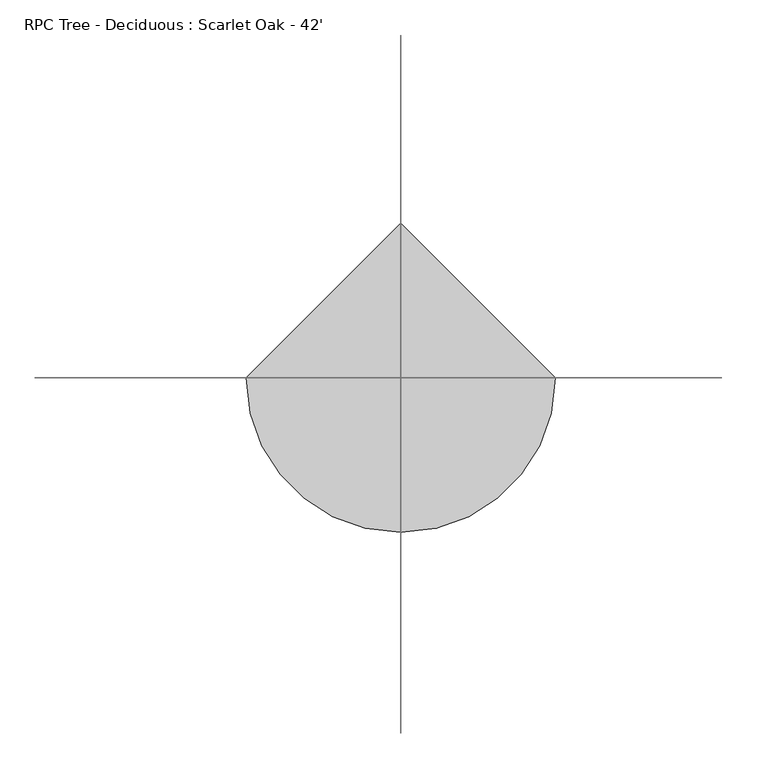
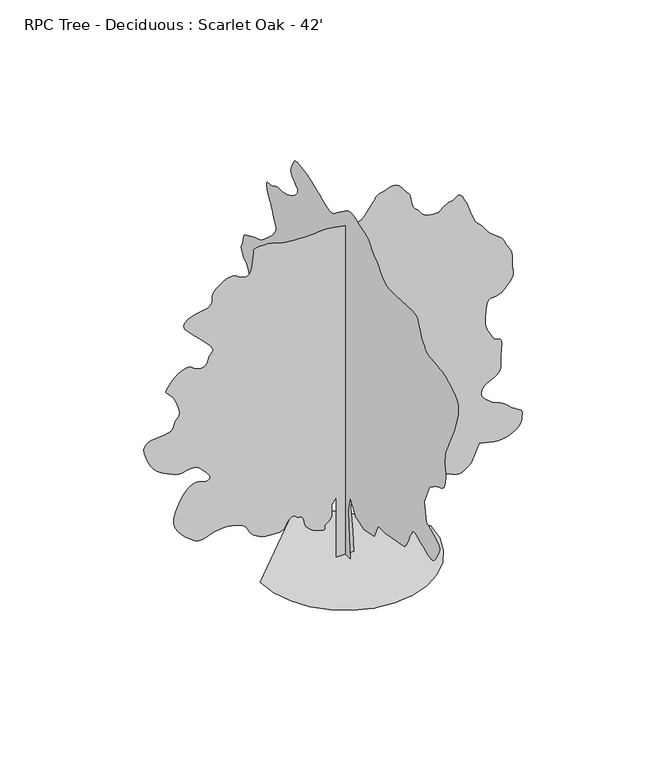
"""IFC4 building model written with IfcOpenShell, lengths in millimetres: geographic element geometry, RPC Tree - Deciduous : Scarlet Oak - 42'."""

import ifcopenshell
import ifcopenshell.guid

model = None  # the IFC model being written
_history = None  # IfcOwnerHistory: only IFC2X3 demands one
_inside = {}  # id of a spatial element -> (the spatial element, [elements in it])
_under = {}  # id of a project, library or spatial element -> (it, [spatial elements below it])
_declared = {}  # id of a project -> (the project, [libraries it declares])
_typed = {}  # id of a type object -> (the type object, [elements of that type])
_made_of = {}  # id of a material, layer set ... -> (it, [elements and type objects made of it])


def new_model(schema):
    """Start an empty IFC model of exactly this schema.

    Asked for "IFC4X3", IfcOpenShell would pick the latest addendum, in which some entities
    have other attributes; the version numbers below select the first issue.
    IFC2X3 requires an IfcOwnerHistory on every rooted entity: one is made here for all.
    """
    global model, _history
    if schema == "IFC4X3":
        model = ifcopenshell.file(schema_version=(4, 3, 0, 0))
    else:
        model = ifcopenshell.file(schema=schema)
    _inside.clear()
    _under.clear()
    _declared.clear()
    _typed.clear()
    _made_of.clear()
    _history = None
    if model.schema == "IFC2X3":
        org = make("IfcOrganization", Name="unknown")
        user = make(
            "IfcPersonAndOrganization",
            ThePerson=make("IfcPerson", FamilyName="unknown"),
            TheOrganization=org,
        )
        app = make(
            "IfcApplication",
            ApplicationDeveloper=org,
            Version="unknown",
            ApplicationFullName="unknown",
            ApplicationIdentifier="unknown",
        )
        _history = make(
            "IfcOwnerHistory",
            OwningUser=user,
            OwningApplication=app,
            ChangeAction="ADDED",
            CreationDate=0,
        )
    return model


def make(cls, **values):
    """One entity of the class cls with the attributes given. An attribute that is None is left unset."""
    return model.create_entity(
        cls, **{name: value for name, value in values.items() if value is not None}
    )


def rooted(cls, **values):
    """An entity with a GlobalId (a new one), such as an element, a storey or a relation."""
    return make(cls, GlobalId=ifcopenshell.guid.new(), OwnerHistory=_history, **values)


def si_unit(unit_type, name, prefix=None):
    """IfcSIUnit, for example si_unit("LENGTHUNIT", "METRE", prefix="MILLI")."""
    return make("IfcSIUnit", UnitType=unit_type, Prefix=prefix, Name=name)


def assignment(units):
    """IfcUnitAssignment: the units of a project."""
    return None if units is None else make("IfcUnitAssignment", Units=units)


def point(xyz):
    """IfcCartesianPoint."""
    return None if xyz is None else make("IfcCartesianPoint", Coordinates=xyz)


def direction(xyz):
    """IfcDirection."""
    return None if xyz is None else make("IfcDirection", DirectionRatios=xyz)


def frame(location, z_axis=None, x_axis=None):
    """IfcAxis2Placement3D, a coordinate frame: its origin and axes. An axis left out is left unset."""
    return make(
        "IfcAxis2Placement3D",
        Location=point(location),
        Axis=direction(z_axis),
        RefDirection=direction(x_axis),
    )


def origin():
    """The frame at (0, 0, 0) with its axes left unset."""
    return frame((0.0, 0.0, 0.0))


def place(relative_to, where):
    """IfcLocalPlacement: puts the frame where relative to a parent placement (None: the world)."""
    return make(
        "IfcLocalPlacement", PlacementRelTo=relative_to, RelativePlacement=where
    )


def context(
    kind, dimensions, precision=None, world=None, true_north=None, identifier=None
):
    """IfcGeometricRepresentationContext, for example the 3D "Model" context."""
    return make(
        "IfcGeometricRepresentationContext",
        ContextIdentifier=identifier,
        ContextType=kind,
        CoordinateSpaceDimension=dimensions,
        Precision=precision,
        WorldCoordinateSystem=world,
        TrueNorth=true_north,
    )


def project(units=None, contexts=None):
    """IfcProject with its units and contexts."""
    return rooted(
        "IfcProject",
        Name="project",
        RepresentationContexts=contexts,
        UnitsInContext=assignment(units),
    )


def spatial(cls, under=None, at=None, **own):
    """A site, building, storey or space (cls), placed at a placement, below another one or the project."""
    s = rooted(cls, ObjectPlacement=at, **own)
    if under is not None:
        _under.setdefault(under.id(), (under, []))[1].append(s)
    return s


def point_list(points):
    """IfcCartesianPointList2D or 3D."""
    cls = (
        "IfcCartesianPointList2D" if len(points[0]) == 2 else "IfcCartesianPointList3D"
    )
    return make(cls, CoordList=points)


def triangles(points, corners, closed=None, point_numbers=None):
    """IfcTriangulatedFaceSet: each triangle names its three corners, points numbered from 1."""
    return make(
        "IfcTriangulatedFaceSet",
        Coordinates=point_list(points),
        Closed=closed,
        CoordIndex=corners,
        PnIndex=point_numbers,
    )


def shape(context_of_items, identifier, shape_type, items):
    """IfcShapeRepresentation: the items that make up one representation, for example the "Body"."""
    return make(
        "IfcShapeRepresentation",
        ContextOfItems=context_of_items,
        RepresentationIdentifier=identifier,
        RepresentationType=shape_type,
        Items=items,
    )


def source(mapping_origin, context_of_items, identifier, shape_type, items):
    """IfcRepresentationMap: a shape defined once, which mapped items show again and again."""
    return make(
        "IfcRepresentationMap",
        MappingOrigin=mapping_origin,
        MappedRepresentation=shape(context_of_items, identifier, shape_type, items),
    )


def transform(
    local_origin,
    x_axis=None,
    y_axis=None,
    z_axis=None,
    scale=None,
    scale2=None,
    scale3=None,
    uniform=True,
):
    """IfcCartesianTransformationOperator3D, or its non-uniform kind. x_axis, y_axis, z_axis: its Axis1, 2, 3."""
    if uniform:
        return make(
            "IfcCartesianTransformationOperator3D",
            Axis1=direction(x_axis),
            Axis2=direction(y_axis),
            LocalOrigin=point(local_origin),
            Scale=scale,
            Axis3=direction(z_axis),
        )
    return make(
        "IfcCartesianTransformationOperator3DnonUniform",
        Axis1=direction(x_axis),
        Axis2=direction(y_axis),
        LocalOrigin=point(local_origin),
        Scale=scale,
        Axis3=direction(z_axis),
        Scale2=scale2,
        Scale3=scale3,
    )


def mapped(mapping_source, mapping_target):
    """IfcMappedItem: shows the shape of a source again, moved by a transform."""
    return make(
        "IfcMappedItem", MappingSource=mapping_source, MappingTarget=mapping_target
    )


def made_of(thing, what):
    """Note that an element or type object is made of a material, layer set ...; save() writes the relation."""
    if what is not None:
        _made_of.setdefault(what.id(), (what, []))[1].append(thing)
    return thing


def element(
    cls,
    number,
    at=None,
    inside=None,
    cuts=None,
    type_object=None,
    material=None,
    context=None,
    identifier="Body",
    shape_type=None,
    held_by="IfcProductDefinitionShape",
    body=None,
    shapes=None,
    **own,
):
    """One element of the class cls, such as IfcWall. Its Tag is "e" and its number.

    at: its placement. inside: the storey or other place that contains it. cuts: it is an
    opening in that element (IfcRelVoidsElement). A single representation is given by context,
    identifier, shape_type and body (its items); several are given by shapes. held_by: the class
    of the entity that holds the representations. save() writes the other relations.
    """
    e = rooted(cls, Tag="e%d" % number, ObjectPlacement=at, **own)
    if body is not None:
        shapes = [shape(context, identifier, shape_type, body)]
    if shapes is not None:
        e.Representation = make(held_by, Representations=shapes)
    if inside is not None:
        _inside.setdefault(inside.id(), (inside, []))[1].append(e)
    if cuts is not None:
        rooted(
            "IfcRelVoidsElement", RelatingBuildingElement=cuts, RelatedOpeningElement=e
        )
    if type_object is not None:
        _typed.setdefault(type_object.id(), (type_object, []))[1].append(e)
    return made_of(e, material)


def aggregate(whole, parts):
    """IfcRelAggregates: a whole, such as a stair, and the parts it consists of."""
    return rooted("IfcRelAggregates", RelatingObject=whole, RelatedObjects=parts)


def save(model, path):
    """Write the relations noted so far, then the file.

    IfcRelAggregates (storeys below a building ...), IfcRelContainedInSpatialStructure (elements
    in a storey), IfcRelDefinesByType, IfcRelAssociatesMaterial and IfcRelDeclares: one each for
    every whole, place, type object, material and project.
    """
    for whole, parts in _under.values():
        aggregate(whole, parts)
    for where, things in _inside.values():
        rooted(
            "IfcRelContainedInSpatialStructure",
            RelatedElements=things,
            RelatingStructure=where,
        )
    for kind, things in _typed.values():
        rooted("IfcRelDefinesByType", RelatedObjects=things, RelatingType=kind)
    for what, things in _made_of.values():
        rooted("IfcRelAssociatesMaterial", RelatedObjects=things, RelatingMaterial=what)
    for by, libraries in _declared.values():
        rooted("IfcRelDeclares", RelatingContext=by, RelatedDefinitions=libraries)
    model.write(path)


def rpc_tree_deciduous_scarlet_oak_42_9b182cbb(model_context):
    return source(origin(), model_context, "Body", "Tessellation", [
        triangles([(0.0176667, 313.3908637, 0.0), (0.0176667, -300.6481277, 0.0), (0.0176667, -201.6098415, 1168.65294), (0.0176667, -181.8016574, 1723.2669067), (0.0176667, -300.6481277, 2238.2675938), (0.0176667, -617.5722605, 1723.2669067), (0.0176667, -1132.5703314, 1564.8060848), (0.0176667, -1726.8001213, 1703.4602669), (0.0176667, -1964.4925896, 2198.6516979), (0.0176667, -2380.4549904, 2198.6516979), (0.0176667, -3529.2988197, 2416.5375263), (0.0176667, -3571.5694954, 2467.5287453), (0.0176667, -3612.8163963, 2518.865728), (0.0176667, -3651.9637161, 2570.8942383), (0.0176667, -3687.9873894, 2623.969487), (0.0176667, -3719.8633507, 2678.4275002), (0.0176667, -3746.5419548, 2734.6266861), (0.0176667, -3766.9988457, 2792.8740028), (0.0176667, -3786.866819, 2852.8877815), (0.0176667, -3811.9324402, 2913.9259163), (0.0176667, -3841.3248322, 2975.8343468), (0.0176667, -3874.1736992, 3038.4340141), (0.0176667, -3909.6343254, 3101.5461502), (0.0176667, -3946.8099632, 3165.016404), (0.0176667, -3984.882058, 3228.6404274), (0.0176667, -4003.0091492, 3249.1996376), (0.0176667, -4028.0747704, 3265.7904854), (0.0176667, -4066.991581, 3274.393158), (0.0176667, -4126.698111, 3271.0392929), (0.0176667, -4214.133181, 3251.7599464), (0.0176667, -4336.2091599, 3212.5358871), (0.0176667, -4499.8648682, 3149.4240417), (0.0176667, -4672.6607162, 3075.1492149), (0.0176667, -4819.8023163, 3008.8625633), (0.0176667, -4944.7714325, 2956.0686928), (0.0176667, -5051.0248306, 2922.3492393), (0.0176667, -5142.0442749, 2913.2343887), (0.0176667, -5221.2603699, 2934.2546173), (0.0176667, -5292.1816223, 2990.9656906), (0.0176667, -5363.7423706, 3080.2954124), (0.0176667, -5437.7099487, 3189.0320892), (0.0176667, -5506.8388687, 3307.4725342), (0.0176667, -5563.8313202, 3425.9129791), (0.0176667, -5601.4168167, 3534.6496559), (0.0176667, -5612.3492889, 3624.0049576), (0.0176667, -5589.3065094, 3684.2236656), (0.0176667, -5533.0052948, 3729.5668282), (0.0176667, -5451.7404877, 3780.0820587), (0.0176667, -5349.7118317, 3834.9496399), (0.0176667, -5231.0155884, 3893.2736961), (0.0176667, -5099.8759186, 3954.2095116), (0.0176667, -4960.4152451, 4016.8603386), (0.0176667, -4816.8068596, 4080.3820427), (0.0176667, -4697.9568466, 4753.8484932), (0.0176667, -4995.0561539, 5447.1064682), (0.0176667, -5004.4270935, 5460.3434509), (0.0176667, -5018.9698105, 5476.4988602), (0.0176667, -5043.9328217, 5498.5690247), (0.0176667, -5084.4629059, 5529.4717896), (0.0176667, -5145.7824188, 5572.1267441), (0.0176667, -5233.1148788, 5629.5290543), (0.0176667, -5351.6064835, 5704.6233078), (0.0176667, -5480.1602646, 5772.6511322), (0.0176667, -5594.1457489, 5817.0984192), (0.0176667, -5693.5885162, 5853.2497009), (0.0176667, -5778.4885666, 5896.340094), (0.0176667, -5848.8209015, 5961.6029709), (0.0176667, -5904.609938, 6064.2717041), (0.0176667, -5945.8312592, 6219.6064087), (0.0176667, -5969.6931747, 6372.1755844), (0.0176667, -5976.5549652, 6470.0056595), (0.0176667, -5971.3064484, 6533.5267822), (0.0176667, -5958.7607025, 6583.1970062), (0.0176667, -5943.8087082, 6639.4476425), (0.0176667, -5931.2885422, 6722.7088394), (0.0176667, -5926.0400253, 6853.4648117), (0.0176667, -5927.8835175, 6997.7129837), (0.0176667, -5935.9737213, 7117.3568436), (0.0176667, -5954.1011032, 7226.6309875), (0.0176667, -5986.0793839, 7339.6950165), (0.0176667, -6035.7496078, 7470.7835266), (0.0176667, -6106.9010788, 7634.1061157), (0.0176667, -6203.3225189, 7843.8473831), (0.0176667, -6294.8797211, 8033.439299), (0.0176667, -6355.9178558, 8147.834642), (0.0176667, -6397.1897552, 8218.5762543), (0.0176667, -6429.4755753, 8277.1819794), (0.0176667, -6463.5019867, 8355.1946594), (0.0176667, -6509.9718246, 8484.1577179), (0.0176667, -6579.6896622, 8695.5634186), (0.0176667, -6654.8094955, 8940.125235), (0.0176667, -6705.3500153, 9150.7373795), (0.0176667, -6723.656456, 9332.2385101), (0.0176667, -6702.0984695, 9489.4934464), (0.0176667, -6633.0980301, 9627.3408463), (0.0176667, -6508.9992096, 9750.6205307), (0.0176667, -6322.1728226, 9864.2211548), (0.0176667, -6140.9019104, 9957.5968506), (0.0176667, -6021.6679092, 10021.8859497), (0.0176667, -5939.1485275, 10064.3101044), (0.0176667, -5868.0487976, 10092.2177032), (0.0176667, -5783.0970062, 10112.8292358), (0.0176667, -5658.9987671, 10133.4396057), (0.0176667, -5470.4567871, 10161.3472046), (0.0176667, -5268.216806, 10183.3400482), (0.0176667, -5111.3717285, 10191.8406921), (0.0176667, -4987.0938492, 10202.3888855), (0.0176667, -4882.5816238, 10230.6290222), (0.0176667, -4784.982058, 10292.127594), (0.0176667, -4681.493898, 10402.5034149), (0.0176667, -4559.2897293, 10577.2962341), (0.0176667, -4452.5756035, 10769.4740387), (0.0176667, -4389.5149178, 10923.9122864), (0.0176667, -4348.2938873, 11044.0165833), (0.0176667, -4307.0469864, 11133.2960175), (0.0176667, -4243.9863007, 11195.2038666), (0.0176667, -4137.2721748, 11233.1992218), (0.0176667, -3965.0652443, 11250.763266), (0.0176667, -3014.2904297, 11191.3378235), (0.0176667, -2839.0363014, 11194.4108917), (0.0176667, -2696.349662, 11194.0004517), (0.0176667, -2575.1186897, 11201.2209412), (0.0176667, -2464.3027794, 11227.1309875), (0.0176667, -2352.7906906, 11282.8694458), (0.0176667, -2229.4985069, 11379.4705261), (0.0176667, -2083.3375156, 11528.0707581), (0.0176667, -1942.4917522, 11678.1569458), (0.0176667, -1836.9835121, 11780.4158203), (0.0176667, -1758.5045815, 11847.7012482), (0.0176667, -1698.7339565, 11892.8147736), (0.0176667, -1649.3606621, 11928.556778), (0.0176667, -1602.0639851, 11967.7555481), (0.0176667, -1548.5328049, 12023.2626251), (0.0176667, -1497.1368141, 12088.8074615), (0.0176667, -1455.0938862, 12149.8444336), (0.0176667, -1412.3621922, 12206.7351471), (0.0176667, -1358.8872585, 12259.7853973), (0.0176667, -1284.6226055, 12309.4044617), (0.0176667, -1179.5189192, 12355.8992981), (0.0176667, -1033.5320452, 12399.6036072), (0.0176667, -869.6434296, 12447.7634583), (0.0176667, -716.8409832, 12501.1206665), (0.0176667, -574.0851983, 12550.3304535), (0.0176667, -440.341763, 12586.0212982), (0.0176667, -314.5660463, 12598.8484222), (0.0176667, -195.7190492, 12579.4414673), (0.0176667, -82.7633712, 12518.4544922), (0.0176667, 511.4674361, 12082.6880676), (0.0176667, 575.7980298, 12024.1335022), (0.0176667, 638.0522604, 11970.7762939), (0.0176667, 705.8469595, 11927.7882202), (0.0176667, 786.8119303, 11900.4189606), (0.0176667, 888.5641497, 11893.8379669), (0.0176667, 1018.7282976, 11913.2460846), (0.0176667, 1184.9289087, 11963.8371826), (0.0176667, 1373.534911, 12038.957016), (0.0176667, 1563.5259304, 12123.4483704), (0.0176667, 1751.4381523, 12209.6791534), (0.0176667, 1933.8071079, 12289.996344), (0.0176667, 2107.1689098, 12356.8213348), (0.0176667, 2268.0542931, 12402.4976166), (0.0176667, 2413.0043118, 12419.4210022), (0.0176667, 2544.8429214, 12428.6634613), (0.0176667, 2667.3156784, 12449.6842712), (0.0176667, 2778.3824455, 12472.4200928), (0.0176667, 2875.9049812, 12486.8599091), (0.0176667, 2957.8610252, 12482.9427063), (0.0176667, 3022.1248352, 12450.606308), (0.0176667, 3066.6488617, 12379.7873749), (0.0176667, 3106.4362587, 12290.8160614), (0.0176667, 3152.1122498, 12208.7582794), (0.0176667, 3195.0232933, 12130.8479187), (0.0176667, 3226.5152664, 12054.318869), (0.0176667, 3237.8831772, 11976.4340881), (0.0176667, 3220.4984825, 11894.3763062), (0.0176667, 3165.7076408, 11805.3794128), (0.0176667, 3081.8572357, 11723.8332275), (0.0176667, 2992.092366, 11659.9534058), (0.0176667, 2909.982843, 11604.7532867), (0.0176667, 2848.9961586, 11549.1938873), (0.0176667, 2822.6759628, 11484.2897095), (0.0176667, 2844.4900383, 11401.0285126), (0.0176667, 2928.0076149, 11290.3713135), (0.0176667, 3043.3244133, 11180.1233917), (0.0176667, 3152.0610901, 11099.7038818), (0.0176667, 3254.9091728, 11042.4550507), (0.0176667, 3352.5598984, 11001.8738068), (0.0176667, 3445.704213, 10971.3035797), (0.0176667, 3535.0595146, 10944.2412781), (0.0176667, 3621.2652992, 10914.0291687), (0.0176667, 3707.3690552, 10890.7561707), (0.0176667, 3795.9049301, 10883.0752441), (0.0176667, 3886.8473442, 10882.333429), (0.0176667, 3980.222168, 10879.8498596), (0.0176667, 4076.0294014, 10866.9715759), (0.0176667, 4174.2690445, 10835.0177124), (0.0176667, 4274.9152267, 10775.3887939), (0.0176667, 4378.9408539, 10722.4152832), (0.0176667, 4481.2000191, 10703.4176056), (0.0176667, 4572.7316414, 10698.9632263), (0.0176667, 4644.5228989, 10689.6684448), (0.0176667, 4687.5362617, 10656.1286316), (0.0176667, 4692.7850693, 10578.9089264), (0.0176667, 4651.2820793, 10438.6546967), (0.0176667, 4589.9369865, 10291.0520782), (0.0176667, 4539.012188, 10191.6093109), (0.0176667, 4494.308812, 10120.561322), (0.0176667, 4451.7053078, 10058.1918732), (0.0176667, 4407.0019318, 9984.7358917), (0.0176667, 4356.0515533, 9880.4538849), (0.0176667, 4294.7320404, 9725.5801987), (0.0176667, 4229.9301819, 9573.2412415), (0.0176667, 4174.1664345, 9477.02444), (0.0176667, 4131.5370598, 9417.880957), (0.0176667, 4106.2412201, 9376.7625366), (0.0176667, 4102.4263367, 9334.6197601), (0.0176667, 4124.265992, 9272.3526306), (0.0176667, 4175.8820274, 9170.9640518), (0.0176667, 4267.7717674, 9036.5728363), (0.0176667, 4396.7095367, 8893.8861969), (0.0176667, 4546.4626053, 8751.5320953), (0.0176667, 4700.6962143, 8618.1908157), (0.0176667, 4843.178215, 8502.5153183), (0.0176667, 4957.5729767, 8413.1858871), (0.0176667, 5027.6233521, 8358.830484), (0.0176667, 5089.8137421, 8324.829071), (0.0176667, 5183.1888565, 8290.4695404), (0.0176667, 5295.279689, 8255.4187729), (0.0176667, 5413.6172333, 8219.3186508), (0.0176667, 5525.7080658, 8181.8354736), (0.0176667, 5619.0831802, 8142.6367035), (0.0176667, 5681.2729889, 8101.3392242), (0.0176667, 5733.3500427, 8067.0308533), (0.0176667, 5799.6622742, 8042.7846588), (0.0176667, 5872.5293381, 8019.2297012), (0.0176667, 5944.3714645, 7986.9950409), (0.0176667, 6007.5606308, 7936.7614792), (0.0176667, 6054.4397461, 7859.1324966), (0.0176667, 6077.431366, 7744.7888947), (0.0176667, 6096.2499847, 7629.9325333), (0.0176667, 6128.5869644, 7548.6938873), (0.0176667, 6163.6888916, 7488.5777893), (0.0176667, 6190.8535126, 7437.1152328), (0.0176667, 6199.277417, 7381.8633728), (0.0176667, 6178.2571884, 7310.3026245), (0.0176667, 6117.0399948, 7209.9889801), (0.0176667, 6041.0492844, 7116.0255295), (0.0176667, 5979.6018723, 7059.8522141), (0.0176667, 5927.8579376, 7023.4183914), (0.0176667, 5880.9526611, 6988.7007431), (0.0176667, 5834.0729645, 6937.699205), (0.0176667, 5782.3290298, 6852.4148758), (0.0176667, 5720.8816177, 6714.7976944), (0.0176667, 5653.9037292, 6576.9502945), (0.0176667, 5592.4557358, 6490.0526917), (0.0176667, 5542.0942749, 6434.6729324), (0.0176667, 5508.3748215, 6391.4034805), (0.0176667, 5496.8278519, 6340.8885406), (0.0176667, 5512.9832611, 6263.6694168), (0.0176667, 5562.4232666, 6140.3897324), (0.0176667, 5628.0954208, 6005.5380798), (0.0176667, 5689.9271118, 5900.8462143), (0.0176667, 5749.0194351, 5817.6361771), (0.0176667, 5806.3450058, 5747.2271027), (0.0176667, 5863.0049194, 5680.9916107), (0.0176667, 5919.9973709, 5610.2499985), (0.0176667, 5978.3728775, 5526.348143), (0.0176667, 6046.1187424, 5443.5985428), (0.0176667, 6124.9511398, 5376.0828964), (0.0176667, 6206.5484848, 5314.8145432), (0.0176667, 6282.6153534, 5250.7556625), (0.0176667, 6344.8057434, 5174.9445923), (0.0176667, 6384.8236496, 5078.3179321), (0.0176667, 6394.3480682, 4951.9151825), (0.0176667, 6402.3615326, 4852.6511833), (0.0176667, 6431.8824051, 4819.9049263), (0.0176667, 6465.5506989, 4818.343103), (0.0176667, 6486.0587494, 4812.6335678), (0.0176667, 6476.0477325, 4767.4183044), (0.0176667, 6418.2611435, 4647.3648766), (0.0176667, 6295.3145782, 4417.1152679), (0.0176667, 6166.7613785, 4158.8557411), (0.0176667, 6089.1579758, 3968.8801277), (0.0176667, 6040.640007, 3832.9270889), (0.0176667, 5999.4186859, 3736.8381866), (0.0176667, 5943.629068, 3666.3782433), (0.0176667, 5851.4579498, 3607.3629501), (0.0176667, 5701.0903839, 3545.5824188), (0.0176667, 5527.4748184, 3495.4511765), (0.0176667, 5374.6748428, 3474.4309479), (0.0176667, 5234.3438736, 3472.8179649), (0.0176667, 5098.1859055, 3480.9087502), (0.0176667, 4957.8549362, 3488.9736649), (0.0176667, 4805.0549606, 3487.3606819), (0.0176667, 4631.4652657, 3466.3404533), (0.0176667, 4458.3362984, 3447.5221252), (0.0176667, 4308.7625793, 3451.5675179), (0.0176667, 4177.2133415, 3467.3900986), (0.0176667, 4058.1328194, 3483.9042068), (0.0176667, 3945.9908272, 3490.0233101), (0.0176667, 3835.2313087, 3474.6614571), (0.0176667, 3720.2984985, 3426.7324059), (0.0176667, 3610.3072472, 3375.7820274), (0.0176667, 3519.3389626, 3349.1034233), (0.0176667, 3449.5190964, 3332.1285873), (0.0176667, 3402.9213593, 3310.3145119), (0.0176667, 3381.6194618, 3269.0679016), (0.0176667, 3387.6874054, 3193.8969086), (0.0176667, 3423.1991913, 3070.1820763), (0.0176667, 3480.4733116, 2938.7610283), (0.0176667, 3549.1923729, 2845.7701927), (0.0176667, 3627.4614326, 2784.8599571), (0.0176667, 3713.3343887, 2749.5789711), (0.0176667, 3804.9171707, 2733.5255905), (0.0176667, 3900.3145454, 2730.2740448), (0.0176667, 3997.6068626, 2733.448851), (0.0176667, 4373.9740059, 2317.4992401), (0.0176667, 4403.4687172, 2270.6632908), (0.0176667, 4431.7603043, 2222.9646034), (0.0176667, 4457.6450615, 2173.5324463), (0.0176667, 4479.868705, 2121.4991398), (0.0176667, 4497.2533997, 2066.004126), (0.0176667, 4508.5698601, 2006.1771091), (0.0176667, 4512.6152527, 1941.1527351), (0.0176667, 4511.9240158, 1873.3554199), (0.0176667, 4507.0847763, 1806.2519577), (0.0176667, 4493.8992439, 1740.5362015), (0.0176667, 4468.2705757, 1676.8969173), (0.0176667, 4425.9996094, 1616.0304291), (0.0176667, 4362.9389236, 1558.6281189), (0.0176667, 4274.9152267, 1505.3836945), (0.0176667, 4190.9622116, 1460.165815), (0.0176667, 4131.9469185, 1424.9973221), (0.0176667, 4081.5854576, 1397.7989822), (0.0176667, 4023.5942299, 1376.4895271), (0.0176667, 3941.7149254, 1358.992194), (0.0176667, 3819.6389465, 1343.2258598), (0.0176667, 3641.0824036, 1327.1137619), (0.0176667, 3437.9721268, 1329.4230686), (0.0176667, 3250.8126205, 1364.996188), (0.0176667, 3076.1221207, 1425.8652924), (0.0176667, 2910.4438614, 1504.0548512), (0.0176667, 2750.3213676, 1591.6024143), (0.0176667, 2592.2472954, 1680.5352127), (0.0176667, 2432.8109516, 1762.8828026), (0.0176667, 2290.6338741, 1837.7823006), (0.0176667, 2180.6808472, 1908.5239128), (0.0176667, 2093.9423916, 1973.376931), (0.0176667, 2021.411063, 2030.6051239), (0.0176667, 1954.0772369, 2078.4780739), (0.0176667, 1882.9309982, 2115.2646366), (0.0176667, 1798.9653385, 2139.2293076), (0.0176667, 1706.624754, 2159.4404285), (0.0176667, 1615.6720207, 2184.5034336), (0.0176667, 1525.0649059, 2211.9936161), (0.0176667, 1433.7664089, 2239.4811825), (0.0176667, 1340.7321167, 2264.5441875), (0.0176667, 1244.9274994, 2284.7553085), (0.0176667, 1145.3130856, 2297.6899841), (0.0176667, 1043.4456116, 2304.4466938), (0.0176667, 941.5755941, 2308.0849892), (0.0176667, 839.7081202, 2309.1244606), (0.0176667, 737.8407188, 2308.0849892), (0.0176667, 635.9732449, 2305.4861652), (0.0176667, 534.1032274, 2301.8480152), (0.0176667, 432.2357898, 2297.6899841), (0.0176667, 234.1596897, 2000.5751255), (0.0176667, 194.5438665, 1544.999445), (287.211575, 0.0006153, 0.0094345), (-307.0182149, 0.0006153, 0.0094345), (-307.0182149, 0.0004871, 2178.8527611), (-465.4815439, 0.0004871, 1960.9695488), (-465.4815439, 0.0005127, 1723.2770805), (-461.8433212, 0.0005127, 1668.1278305), (-461.8433212, 0.0005127, 1613.1500816), (-469.1197666, 0.0005127, 1558.5205673), (-487.308264, 0.0005384, 1504.4107887), (-520.0521955, 0.0005384, 1450.9948631), (-570.9872043, 0.0005384, 1398.4416756), (-643.748933, 0.0005384, 1346.9305756), (-700.7467621, 0.0005384, 1293.4557873), (-716.5132416, 0.0005384, 1239.2870007), (-712.8750189, 0.0005384, 1191.0121857), (-711.6614302, 0.0005384, 1155.206159), (-734.7042824, 0.0005384, 1138.4590708), (-803.8278248, 0.0005384, 1147.3536587), (-940.8638643, 0.0005384, 1188.4698263), (-1097.1892788, 0.0005384, 1252.5136642), (-1214.0141247, 0.0005384, 1324.8708755), (-1297.9209217, 0.0005384, 1404.1613846), (-1355.4973492, 0.0005384, 1488.9925438), (-1393.3235287, 0.0005127, 1577.9815887), (-1417.9820526, 0.0005127, 1669.7434296), (-1436.0578388, 0.0005127, 1762.8929764), (-1440.6767429, 0.0005127, 1788.2427372), (-1447.5485619, 0.0005127, 1812.9011158), (-1458.9240303, 0.0005127, 1836.1770206), (-1477.0588245, 0.0005127, 1857.3687504), (-1504.1983017, 0.0005127, 1875.7903004), (-1542.6030796, 0.0005127, 1890.7476723), (-1594.5186607, 0.0005127, 1901.5471584), (-1646.4342419, 0.0005127, 1919.331102), (-1687.2611103, 0.0005127, 1949.2458458), (-1722.8930923, 0.0004871, 1981.5852962), (-1759.2163113, 0.0004871, 2006.6483013), (-1802.1247387, 0.0004871, 2014.733709), (-1857.5044979, 0.0004871, 1996.138187), (-1931.2494152, 0.0005127, 1941.1604382), (-1996.0996719, 0.0005127, 1864.2407146), (-2032.88638, 0.0005127, 1789.0516994), (-2059.6238468, 0.0005127, 1719.7541851), (-2094.3289959, 0.0005127, 1660.5031506), (-2155.0238377, 0.0005127, 1615.4620045), (-2259.7204994, 0.0005127, 1588.7809296), (-2426.4408463, 0.0005127, 1584.6230438), (-2610.6557648, 0.0005127, 1596.8664825), (-2760.2297745, 0.0005127, 1617.0776035), (-2881.7168358, 0.0005127, 1645.9528759), (-2981.7488113, 0.0005127, 1684.1810658), (-3066.8793709, 0.0005127, 1732.4584969), (-3143.6633469, 0.0005127, 1791.4788769), (-3218.7576004, 0.0005127, 1861.9312626), (-3282.4327835, 0.0005127, 1939.1966045), (-3328.1343544, 0.0004871, 2016.8126518), (-3366.8721062, 0.0004871, 2092.6929039), (-3409.782859, 0.0004871, 2164.7633595), (-3467.9278564, 0.0004871, 2230.9424595), (-3552.4183388, 0.0004871, 2289.1538773), (-3674.3152588, 0.0004871, 2337.3161991), (-3796.8778358, 0.0004871, 2373.9261738), (-3885.797699, 0.0004615, 2399.7981411), (-3956.0271332, 0.0004615, 2416.3148655), (-4022.4419746, 0.0004615, 2424.8611462), (-4099.9171875, 0.0004615, 2426.8249798), (-4203.4053474, 0.0004615, 2423.5911655), (-4347.7817093, 0.0004615, 2416.5452293), (-4506.5217293, 0.0004615, 2391.541087), (-4647.6209656, 0.0004871, 2345.0533722), (-4777.6083801, 0.0004871, 2294.4077717), (-4903.0896744, 0.0004871, 2256.9298267), (-5030.6702591, 0.0004871, 2249.9426079), (-5166.8793869, 0.0004871, 2290.7694763), (-5318.3480484, 0.0004615, 2396.7385895), (-5476.8319794, 0.0004615, 2538.4523232), (-5623.153862, 0.0004615, 2679.118737), (-5747.6625412, 0.0004358, 2825.0057625), (-5840.6277969, 0.0004358, 2982.3118584), (-5892.3717316, 0.0004358, 3157.2843178), (-5893.1908676, 0.0004102, 3356.1698524), (-5833.3561478, 0.0004102, 3585.1904663), (-5733.2221436, 0.0003846, 3816.1824715), (-5621.6434891, 0.0003846, 4014.2744499), (-5501.7694107, 0.0003589, 4175.6259384), (-5376.6973938, 0.0003589, 4296.4217628), (-5249.5266678, 0.0003589, 4372.8729103), (-5123.4052963, 0.0003589, 4401.1900772), (-5001.4313461, 0.0003589, 4377.5072205), (-4886.3965073, 0.0003589, 4337.6686638), (-4784.5469101, 0.0003589, 4320.6679573), (-4704.1526894, 0.0003589, 4327.6064873), (-4653.5607193, 0.0003589, 4359.4824486), (-4641.0920036, 0.0003589, 4417.3457771), (-4675.0419662, 0.0003589, 4502.2458275), (-4763.7313202, 0.0003333, 4615.2072464), (-4867.1683205, 0.0003333, 4728.5014938), (-4946.0004272, 0.0003333, 4815.808374), (-5009.573291, 0.0003333, 4880.2515335), (-5067.2575607, 0.0003333, 4924.9546188), (-5128.4235947, 0.0003333, 4953.0156967), (-5202.3911728, 0.0003076, 4967.5839935), (-5298.5568146, 0.0003076, 4971.7319962), (-5397.1804459, 0.0003333, 4962.437796), (-5478.8545303, 0.0003333, 4941.0077087), (-5553.2313858, 0.0003333, 4917.171373), (-5630.0412323, 0.0003333, 4900.5805252), (-5718.9613861, 0.0003333, 4900.9903839), (-5829.7209045, 0.0003333, 4928.0782654), (-5972.0232651, 0.0003076, 4991.5488098), (-6123.0309082, 0.0003076, 5067.4877792), (-6256.0140701, 0.0003076, 5133.3645721), (-6374.8126328, 0.0003076, 5201.008699), (-6483.1909012, 0.0003076, 5282.1450256), (-6585.0149185, 0.0003076, 5388.5519028), (-6684.0484085, 0.000282, 5532.0576782), (-6784.1312531, 0.000282, 5724.4401215), (-6866.8808533, 0.0002564, 5924.068634), (-6912.5565536, 0.0002564, 6084.5495361), (-6922.9006897, 0.0002564, 6210.3889481), (-6899.6271103, 0.0002307, 6306.0679916), (-6844.4775696, 0.0002307, 6376.118367), (-6759.1938217, 0.0002307, 6425.0206146), (-6645.4641357, 0.0002307, 6457.3064346), (-6511.2008194, 0.0002307, 6475.8430939), (-6369.3338974, 0.0002307, 6486.7755661), (-6229.1564072, 0.0002307, 6499.3980515), (-6100.090448, 0.0002307, 6523.1320679), (-5991.4813797, 0.0002307, 6567.3229752), (-5912.6495636, 0.0002307, 6641.2911346), (-5872.9641953, 0.0002051, 6754.4313217), (-5843.6485428, 0.0002051, 6863.6804672), (-5798.3565399, 0.0002051, 6934.8313568), (-5750.3251694, 0.0002051, 6990.3907562), (-5712.6629333, 0.0002051, 7052.8625244), (-5698.5812347, 0.0001795, 7144.8034241), (-5721.2141556, 0.0001795, 7288.7190582), (-5793.7481003, 0.0001795, 7507.1144485), (-5896.4679932, 0.0001538, 7722.232132), (-5994.7079269, 0.0001538, 7857.6477036), (-6079.0702194, 0.0001538, 7937.9904739), (-6140.2362534, 0.0001282, 7987.8141769), (-6168.8095093, 0.0001282, 8031.7492859), (-6155.4702072, 0.0001282, 8094.4262741), (-6090.8474075, 0.0001282, 8200.3977127), (-5986.6938812, 0.0001282, 8332.6384781), (-5866.2308853, 0.0001025, 8453.101474), (-5737.4468857, 0.0001025, 8554.8481705), (-5608.304187, 0.0001025, 8630.9667801), (-5486.816835, 0.0001025, 8674.4920303), (-5380.8965561, 0.0001025, 8678.5377136), (-5298.5568146, 0.0001025, 8636.1641373), (-5217.8297653, 0.0001025, 8572.9755524), (-5118.386998, 0.0001025, 8523.663446), (-5010.6232269, 0.0001025, 8494.7832321), (-4904.9331665, 0.0001025, 8492.93974), (-4811.7374016, 0.0001025, 8524.713382), (-4741.4053574, 0.0001025, 8596.6584091), (-4704.3320389, 0.0001025, 8715.3802322), (-4670.3564964, 0.0001025, 8828.5721603), (-4616.9995789, 7.69e-05, 8895.677948), (-4566.0747803, 7.69e-05, 8940.9449524), (-4539.3961761, 7.69e-05, 8988.6432037), (-4558.8034218, 7.69e-05, 9063.0206406), (-4646.110302, 7.69e-05, 9188.3484558), (-4823.1820518, 5.13e-05, 9388.8472641), (-5045.2129761, 5.13e-05, 9615.3328583), (-5243.6892334, 2.56e-05, 9806.1281891), (-5404.7584717, 2.56e-05, 9966.78815), (-5514.5197952, 2.56e-05, 10102.8437988), (-5559.1717209, 0.0, 10219.8506104), (-5524.8121902, 0.0, 10323.3384796), (-5397.5897232, 0.0, 10418.8384644), (-5227.9175217, 0.0, 10492.422345), (-5075.9366821, 0.0, 10534.4628021), (-4942.313443, 0.0, 10557.0951416), (-4827.7393318, -2.56e-05, 10572.4569946), (-4732.9050041, -2.56e-05, 10592.6580872), (-4658.527858, -2.56e-05, 10629.8593048), (-4605.2732597, -2.56e-05, 10696.1459564), (-4578.7225548, -2.56e-05, 10774.5690765), (-4574.6774529, -2.56e-05, 10843.2881378), (-4579.2858925, -2.56e-05, 10907.1679596), (-4578.7225548, -2.56e-05, 10971.0477814), (-4559.0850906, -5.13e-05, 11039.7668427), (-4506.5217293, -5.13e-05, 11118.1899628), (-4407.2068611, -5.13e-05, 11211.1552185), (-4285.6427696, -5.13e-05, 11303.1472778), (-4174.4736832, -5.13e-05, 11374.7080261), (-4071.9840088, -7.69e-05, 11424.7619476), (-3976.4072845, -7.69e-05, 11452.3114288), (-3886.0282082, -7.69e-05, 11456.3053711), (-3799.1053162, -7.69e-05, 11435.6694214), (-3713.9488861, -5.13e-05, 11389.4303833), (-3626.1556984, -5.13e-05, 11332.8977875), (-3535.6225616, -5.13e-05, 11288.8353607), (-3446.8053085, -5.13e-05, 11267.2773743), (-3364.2091873, -5.13e-05, 11278.3115845), (-3292.3667702, -5.13e-05, 11331.9501709), (-3235.783596, -7.69e-05, 11438.2808899), (-3198.9404961, -7.69e-05, 11607.3135956), (-3176.9473618, -7.69e-05, 11788.8141449), (-3161.1759407, -0.0001025, 11929.0683746), (-3150.6018768, -0.0001025, 12032.966684), (-3144.2011047, -0.0001025, 12105.3204071), (-3140.8981087, -0.0001025, 12150.9966888), (-3139.6946938, -0.0001025, 12174.8591858), (-3139.5156349, -0.0001025, 12181.7203949), (-3113.477108, -0.0001025, 12185.7666595), (-3042.7354958, -0.0001025, 12194.6765808), (-2938.3767494, -0.0001025, 12203.5609222), (-2811.5129814, -0.0001025, 12207.6060242), (-2673.2045631, -0.0001025, 12201.9470673), (-2534.5452942, -0.0001025, 12181.7203949), (-2406.6342064, -0.0001025, 12142.1123474), (-2289.3460167, -0.0001025, 12098.0499207), (-2171.7120632, -0.0001025, 12066.1227997), (-2048.5351341, -0.0001025, 12043.872995), (-1914.6149654, -0.0001025, 12028.921582), (-1764.7594322, -0.0001025, 12018.8338257), (-1593.7659451, -0.0001025, 12011.1528992), (-1396.4394722, -0.0001025, 12003.4719727), (-1205.9875071, -0.0001025, 12002.3708771), (-1049.1423569, -0.0001025, 12011.6644958), (-911.0079105, -0.0001025, 12024.772998), (-776.6858768, -0.0001025, 12035.1165527), (-631.2776012, -0.0001025, 12036.0897491), (-459.8795603, -0.0001025, 12021.1371735), (-247.5965149, -0.0001025, 11983.6545776), (-33.003293, -0.0001025, 11939.0793915), (140.0111032, -0.0001025, 11908.3556854), (278.3759043, -0.0001025, 11893.2240509), (389.0226934, -0.0001025, 11895.4006622), (478.8797087, -0.0001025, 11916.6761078), (554.8751063, -0.0001025, 11958.7165649), (623.9422932, -0.0001025, 12023.2626251), (921.0572245, -0.0001282, 12399.6036072), (965.640041, -0.0001282, 12457.6465759), (1001.2131603, -0.0001282, 12512.2327789), (1033.3195581, -0.0001282, 12562.2867004), (1067.507515, -0.0001282, 12606.8107269), (1109.3175356, -0.0001282, 12644.7549225), (1164.2952845, -0.0001282, 12675.0693512), (1237.9812664, -0.0001282, 12696.729657), (1328.2991547, -0.0001538, 12721.5641876), (1426.9329597, -0.0001538, 12754.7203033), (1530.070269, -0.0001538, 12785.0858917), (1633.9040474, -0.0001538, 12801.6), (1734.6167953, -0.0001538, 12793.1760956), (1828.3987164, -0.0001538, 12748.7032288), (1911.4427753, -0.0001282, 12657.1216095), (1985.1850765, -0.0001282, 12552.6605438), (2052.6930199, -0.0001282, 12471.3957367), (2112.5788994, -0.0001282, 12405.0323456), (2163.4550091, -0.0001282, 12345.2743652), (2203.9362591, -0.0001282, 12283.7757935), (2232.6374142, -0.0001025, 12212.2138824), (2248.1709137, -0.0001025, 12122.2961151), (2258.9703999, -0.0001025, 12029.1006409), (2273.9277718, -0.0001025, 11951.4972382), (2292.3491764, -0.0001025, 11886.8744385), (2313.5410515, -7.69e-05, 11832.6463531), (2336.8143402, -7.69e-05, 11786.2026764), (2361.4727188, -7.69e-05, 11744.9819366), (2386.8250957, -7.69e-05, 11706.3459229), (2412.4640831, -7.69e-05, 11688.9621002), (2439.1453033, -7.69e-05, 11669.1447052), (2467.9025597, -7.69e-05, 11644.4892334), (2499.7811371, -7.69e-05, 11612.5621124), (2535.8152748, -7.69e-05, 11570.9309326), (2577.0389214, -7.69e-05, 11517.164447), (2624.5072449, -7.69e-05, 11448.8546631), (2694.8648689, -5.13e-05, 11383.9249054), (2794.3076363, -5.13e-05, 11339.4776184), (2908.2931206, -5.13e-05, 11311.6223419), (3022.2786049, -5.13e-05, 11296.6186066), (3121.7213722, -5.13e-05, 11290.601532), (3192.0789963, -5.13e-05, 11289.8073944), (3218.7576004, -5.13e-05, 11290.3968933), (3232.429731, -5.13e-05, 11304.6576508), (3270.0408073, -5.13e-05, 11341.4240112), (3326.3420219, -5.13e-05, 11391.7337311), (3396.1621788, -7.69e-05, 11446.5245728), (3474.2774689, -7.69e-05, 11496.8354553), (3555.5419853, -7.69e-05, 11533.6273956), (3634.7072113, -7.69e-05, 11547.8881531), (3705.6790421, -7.69e-05, 11565.2731384), (3768.3301598, -7.69e-05, 11604.4707458), (3826.500737, -7.69e-05, 11646.1019257), (3883.9542068, -7.69e-05, 11670.7829773), (3944.5313232, -7.69e-05, 11659.0569489), (4012.0469696, -7.69e-05, 11591.5413025), (4090.2904495, -7.69e-05, 11448.8546631), (4163.9763588, -5.13e-05, 11281.2055939), (4218.94655, -5.13e-05, 11145.7894409), (4260.756498, -5.13e-05, 11033.5707092), (4294.9366791, -2.56e-05, 10935.5871552), (4327.0431496, -2.56e-05, 10842.7765411), (4362.631675, -2.56e-05, 10746.1754608), (4407.2068611, -2.56e-05, 10636.7216766), (4453.011042, 0.0, 10540.6833527), (4492.2095215, 0.0, 10479.6452179), (4530.3839355, 0.0, 10437.682663), (4573.0644699, 0.0, 10398.8164307), (4625.7813103, 0.0, 10347.1230743), (4694.0908035, 0.0, 10266.6779846), (4783.5481339, 0.0, 10141.5298096), (4893.6675751, 2.56e-05, 10002.2487762), (5014.5404297, 2.56e-05, 9885.8303009), (5137.4869949, 2.56e-05, 9786.0294159), (5253.8537292, 5.13e-05, 9696.6488251), (5354.9603485, 5.13e-05, 9611.4156555), (5432.1794724, 5.13e-05, 9524.0831955), (5476.8319794, 5.13e-05, 9428.4553116), (5511.8827469, 5.13e-05, 9334.6709198), (5560.7844131, 7.69e-05, 9250.5900055), (5615.6008347, 7.69e-05, 9166.5090912), (5668.3179657, 7.69e-05, 9072.724118), (5710.9985001, 7.69e-05, 8959.5583511), (5735.6545532, 0.0001025, 8817.2554092), (5734.3232391, 0.0001025, 8636.1641373), (5731.6094513, 0.0001025, 8462.1137146), (5746.5614456, 0.0001282, 8335.1732071), (5762.8964951, 0.0001282, 8237.0100128), (5764.3557083, 0.0001282, 8149.2171158), (5734.6046173, 0.0001282, 8053.4863312), (5657.4110733, 0.0001538, 7931.3850632), (5516.4400269, 0.0001538, 7764.6057083), (5349.148494, 0.0001538, 7624.5816971), (5204.0294449, 0.0001538, 7568.3828018), (5081.4159988, 0.0001538, 7556.195755), (4981.691272, 0.0001538, 7548.1817093), (4905.163385, 0.0001795, 7504.4518204), (4852.2160355, 0.0001795, 7385.2172379), (4823.156472, 0.0001795, 7150.5896988), (4812.3007393, 0.0002051, 6890.9474075), (4813.9393021, 0.0002051, 6708.2178635), (4828.3538292, 0.0002307, 6579.9198807), (4855.9797592, 0.0002307, 6483.4728607), (4897.0981796, 0.0002307, 6396.396199), (4952.0686615, 0.0002307, 6296.1342957), (5021.2481598, 0.0002564, 6160.206546), (5100.1828766, 0.0002564, 6041.9969009), (5179.8344101, 0.0002564, 5988.229834), (5253.5717697, 0.0002564, 5966.3393097), (5314.840123, 0.0002564, 5943.7575485), (5357.0602203, 0.0002564, 5887.9167709), (5373.6254883, 0.000282, 5766.2247803), (5357.9816757, 0.000282, 5546.1649567), (5336.7312286, 0.0003076, 5303.5495331), (5333.4796829, 0.0003076, 5126.0935043), (5337.1916656, 0.0003076, 4998.8710373), (5336.7312286, 0.0003333, 4907.0068771), (5321.0106766, 0.0003333, 4835.574028), (5278.9702194, 0.0003333, 4769.6713646), (5199.5233246, 0.0003333, 4694.423632), (5103.537323, 0.0003333, 4623.8610786), (5018.6366913, 0.0003333, 4576.1622459), (4943.7988174, 0.0003333, 4542.6733017), (4877.9726028, 0.0003589, 4514.7145432), (4820.109565, 0.0003589, 4483.6580086), (4769.1847664, 0.0003589, 4440.7981247), (4724.1232727, 0.0003589, 4377.5072205), (4688.3301086, 0.0003589, 4304.2308792), (4668.1034363, 0.0003589, 4235.1022499), (4666.951181, 0.0003589, 4167.0232658), (4688.3301086, 0.0003846, 4096.8447006), (4735.6702423, 0.0003846, 4021.4946487), (4812.4797981, 0.0003846, 3937.7977226), (4922.2152512, 0.0003846, 3842.7075966), (5038.5046646, 0.0003846, 3759.3690788), (5137.1538757, 0.0003846, 3704.7831665), (5224.6915558, 0.0004102, 3666.5061424), (5307.748114, 0.0004102, 3632.0442924), (5392.8533844, 0.0004102, 3588.9030304), (5486.6377762, 0.0004102, 3524.6133499), (5595.6561218, 0.0004102, 3426.7324059), (5711.4083588, 0.0004102, 3325.6252052), (5818.1221939, 0.0004102, 3253.27061), (5911.6763672, 0.0004358, 3199.6064438), (5987.8972961, 0.0004358, 3154.6213989), (6042.6369781, 0.0004358, 3108.254171), (6071.7474106, 0.0004358, 3050.4420021), (6071.0561737, 0.0004358, 2971.148877), (6059.6888443, 0.0004358, 2881.1282089), (6052.801474, 0.0004615, 2796.6374359), (6040.3836273, 0.0004615, 2715.961837), (6012.3737091, 0.0004615, 2637.3855286), (5958.7351227, 0.0004615, 2559.1269333), (5869.4056915, 0.0004615, 2479.4908058), (5734.3232391, 0.0004615, 2396.7385895), (5573.023201, 0.0004871, 2329.7503819), (5411.7481613, 0.0004871, 2294.9863701), (5250.4481232, 0.0004871, 2287.0749344), (5089.148085, 0.0004871, 2300.6446003), (4927.8736267, 0.0004871, 2330.3265095), (4766.5732979, 0.0004871, 2370.7513676), (4605.2732597, 0.0004615, 2416.5452293), (4327.9648956, 0.0005127, 1802.5088722), (4260.0141014, 0.0005127, 1743.6034561), (4191.6790283, 0.0005127, 1687.8192158), (4122.6785889, 0.0005127, 1638.2719494), (4052.6282135, 0.0005127, 1598.0774551), (3981.1950737, 0.0005127, 1570.3595249), (3908.0213425, 0.0005127, 1558.2338116), (3832.7733192, 0.0005127, 1564.816404), (3771.4538063, 0.0005127, 1579.7711597), (3732.639315, 0.0005127, 1592.3039703), (3704.9366455, 0.0005127, 1604.8367809), (3676.8755676, 0.0005127, 1619.7915367), (3637.0114311, 0.0005127, 1639.6007927), (3573.9507454, 0.0005127, 1666.6838779), (3476.2488602, 0.0005127, 1703.4704407), (3348.9752335, 0.0005127, 1756.8865116), (3209.9244186, 0.0005127, 1827.6281239), (3066.7000214, 0.0005127, 1908.7645958), (2926.957679, 0.0004871, 1993.3652458), (2798.2759987, 0.0004871, 2074.5018631), (2688.335907, 0.0004871, 2145.2434753), (2604.716011, 0.0004871, 2198.6620171), (2533.9101585, 0.0004871, 2245.7258595), (2457.9147972, 0.0004871, 2301.1054733), (2377.5848167, 0.0004871, 2363.4185303), (2293.7932743, 0.0004615, 2431.2722374), (2207.4004372, 0.0004615, 2503.2838303), (2119.2767464, 0.0004615, 2578.0629868), (2030.2877014, 0.0004615, 2654.2324654), (2010.4784454, 0.0004358, 2951.3576431), (1614.3253006, 0.0004358, 2990.9656906), (901.2479685, 0.0004358, 2931.5408295), (425.8657207, 0.0004615, 2674.049279), (227.7880946, 0.0004871, 2198.6620171), (188.1730163, 0.0005127, 1644.0454342), (247.5954975, 0.000564, 732.8941458), (-2924.8072289, 0.0, 0.0229709), (-2847.485495, -670.1739916, 0.0229709), (-2627.2724831, -1285.6237072, 0.0229709), (-2281.8083954, -1828.7110519, 0.0229709), (-1828.7110519, -2281.8083954, 0.0229709), (-1285.6237072, -2627.2724831, 0.0229709), (-670.1739916, -2847.485495, 0.0229709), (0.0001278, -2924.8072289, 0.0229709), (670.1739916, -2847.485495, 0.0229709), (1285.6237072, -2627.2724831, 0.0229709), (1828.7110519, -2281.8083954, 0.0229709), (2281.8083954, -1828.7110519, 0.0229709), (2627.2724831, -1285.6237072, 0.0229709), (2847.485495, -670.1739916, 0.0229709), (2924.8072289, 0.0002564, 0.0229709), (-0.0003835, 2924.8072289, 0.0229709)], [[1, 2, 3], [368, 1, 3], [368, 3, 4], [367, 368, 4], [367, 4, 5], [277, 278, 279], [366, 367, 5], [276, 277, 279], [276, 279, 280], [7, 8, 9], [6, 7, 9], [5, 6, 9], [315, 316, 317], [201, 202, 203], [200, 201, 203], [200, 203, 204], [199, 200, 204], [199, 204, 205], [198, 199, 205], [198, 205, 206], [198, 206, 207], [197, 198, 207], [197, 207, 208], [275, 276, 280], [196, 197, 208], [195, 196, 208], [194, 195, 208], [194, 208, 209], [193, 194, 209], [192, 193, 209], [192, 209, 210], [191, 192, 210], [191, 210, 211], [191, 211, 212], [190, 191, 212], [190, 212, 213], [190, 213, 214], [189, 190, 214], [189, 214, 215], [188, 189, 215], [187, 188, 215], [186, 187, 215], [10, 11, 12], [314, 315, 317], [10, 12, 13], [10, 13, 14], [10, 14, 15], [10, 15, 16], [10, 16, 17], [10, 17, 18], [10, 18, 19], [10, 19, 20], [10, 20, 21], [10, 21, 22], [185, 186, 215], [185, 215, 216], [275, 280, 281], [10, 22, 23], [167, 168, 169], [166, 167, 169], [165, 166, 169], [165, 169, 170], [164, 165, 170], [164, 170, 171], [163, 164, 171], [163, 171, 172], [163, 172, 173], [163, 173, 174], [163, 174, 175], [163, 175, 176], [163, 176, 177], [163, 177, 178], [163, 178, 179], [163, 179, 180], [162, 163, 180], [161, 162, 180], [160, 161, 180], [159, 160, 180], [159, 180, 181], [158, 159, 181], [157, 158, 181], [156, 157, 181], [156, 181, 182], [155, 156, 182], [154, 155, 182], [154, 182, 183], [9, 10, 23], [9, 23, 24], [9, 24, 25], [45, 46, 47], [44, 45, 47], [44, 47, 48], [43, 44, 48], [43, 48, 49], [42, 43, 49], [42, 49, 50], [41, 42, 50], [40, 41, 50], [40, 50, 51], [39, 40, 51], [38, 39, 51], [37, 38, 51], [36, 37, 51], [35, 36, 51], [34, 35, 51], [33, 34, 51], [33, 51, 52], [32, 33, 52], [32, 52, 53], [31, 32, 53], [30, 31, 53], [29, 30, 53], [28, 29, 53], [28, 53, 54], [27, 28, 54], [26, 27, 54], [5, 9, 25], [5, 25, 26], [5, 26, 54], [5, 54, 55], [366, 5, 55], [365, 366, 55], [364, 365, 55], [363, 364, 55], [362, 363, 55], [361, 362, 55], [361, 55, 56], [153, 154, 183], [153, 183, 184], [313, 314, 317], [360, 361, 56], [184, 185, 216], [153, 184, 216], [152, 153, 216], [152, 216, 217], [243, 244, 245], [242, 243, 245], [242, 245, 246], [241, 242, 246], [241, 246, 247], [241, 247, 248], [240, 241, 248], [240, 248, 249], [240, 249, 250], [239, 240, 250], [239, 250, 251], [238, 239, 251], [237, 238, 251], [236, 237, 251], [235, 236, 251], [234, 235, 251], [233, 234, 251], [232, 233, 251], [231, 232, 251], [230, 231, 251], [229, 230, 251], [228, 229, 251], [228, 251, 252], [227, 228, 252], [226, 227, 252], [226, 252, 253], [226, 253, 254], [226, 254, 255], [226, 255, 256], [226, 256, 257], [225, 226, 257], [224, 225, 257], [223, 224, 257], [222, 223, 257], [222, 257, 258], [221, 222, 258], [220, 221, 258], [115, 116, 117], [114, 115, 117], [114, 117, 118], [113, 114, 118], [113, 118, 119], [112, 113, 119], [111, 112, 119], [110, 111, 119], [152, 217, 218], [313, 317, 318], [313, 318, 319], [313, 319, 320], [313, 320, 321], [313, 321, 322], [313, 322, 323], [313, 323, 324], [313, 324, 325], [313, 325, 326], [313, 326, 327], [313, 327, 328], [313, 328, 329], [313, 329, 330], [313, 330, 331], [313, 331, 332], [313, 332, 333], [313, 333, 334], [313, 334, 335], [313, 335, 336], [313, 336, 337], [313, 337, 338], [313, 338, 339], [313, 339, 340], [313, 340, 341], [312, 313, 341], [312, 341, 342], [312, 342, 343], [311, 312, 343], [311, 343, 344], [311, 344, 345], [310, 311, 345], [310, 345, 346], [310, 346, 347], [310, 347, 348], [309, 310, 348], [309, 348, 349], [309, 349, 350], [308, 309, 350], [308, 350, 351], [307, 308, 351], [307, 351, 352], [307, 352, 353], [307, 353, 354], [307, 354, 355], [307, 355, 356], [307, 356, 357], [307, 357, 358], [306, 307, 358], [306, 358, 359], [306, 359, 360], [306, 360, 56], [305, 306, 56], [305, 56, 57], [304, 305, 57], [303, 304, 57], [302, 303, 57], [301, 302, 57], [301, 57, 58], [301, 58, 59], [110, 119, 120], [109, 110, 120], [109, 120, 121], [301, 59, 60], [300, 301, 60], [300, 60, 61], [151, 152, 218], [109, 121, 122], [300, 61, 62], [145, 146, 147], [144, 145, 147], [143, 144, 147], [143, 147, 148], [142, 143, 148], [141, 142, 148], [140, 141, 148], [140, 148, 149], [139, 140, 149], [138, 139, 149], [137, 138, 149], [136, 137, 149], [135, 136, 149], [134, 135, 149], [133, 134, 149], [132, 133, 149], [132, 149, 150], [131, 132, 150], [130, 131, 150], [129, 130, 150], [128, 129, 150], [127, 128, 150], [126, 127, 150], [126, 150, 151], [126, 151, 218], [125, 126, 218], [124, 125, 218], [123, 124, 218], [123, 218, 219], [122, 123, 219], [109, 122, 219], [108, 109, 219], [108, 219, 220], [108, 220, 258], [108, 258, 259], [108, 259, 260], [108, 260, 261], [108, 261, 262], [107, 108, 262], [107, 262, 263], [107, 263, 264], [106, 107, 264], [106, 264, 265], [106, 265, 266], [106, 266, 267], [106, 267, 268], [105, 106, 268], [104, 105, 268], [103, 104, 268], [102, 103, 268], [101, 102, 268], [100, 101, 268], [99, 100, 268], [98, 99, 268], [97, 98, 268], [96, 97, 268], [95, 96, 268], [94, 95, 268], [93, 94, 268], [92, 93, 268], [91, 92, 268], [90, 91, 268], [89, 90, 268], [88, 89, 268], [87, 88, 268], [86, 87, 268], [85, 86, 268], [84, 85, 268], [83, 84, 268], [82, 83, 268], [81, 82, 268], [80, 81, 268], [79, 80, 268], [78, 79, 268], [77, 78, 268], [76, 77, 268], [75, 76, 268], [74, 75, 268], [73, 74, 268], [72, 73, 268], [71, 72, 268], [70, 71, 268], [69, 70, 268], [68, 69, 268], [67, 68, 268], [66, 67, 268], [65, 66, 268], [64, 65, 268], [63, 64, 268], [62, 63, 268], [300, 62, 268], [299, 300, 268], [298, 299, 268], [297, 298, 268], [296, 297, 268], [295, 296, 268], [294, 295, 268], [293, 294, 268], [292, 293, 268], [291, 292, 268], [290, 291, 268], [289, 290, 268], [288, 289, 268], [287, 288, 268], [286, 287, 268], [285, 286, 268], [284, 285, 268], [283, 284, 268], [282, 283, 268], [281, 282, 268], [275, 281, 268], [275, 268, 269], [274, 275, 269], [274, 269, 270], [274, 270, 271], [273, 274, 271], [272, 273, 271], [802, 369, 370], [802, 370, 371], [801, 802, 371], [800, 801, 371], [575, 576, 577], [799, 800, 371], [574, 575, 577], [383, 384, 385], [383, 385, 386], [382, 383, 386], [382, 386, 387], [381, 382, 387], [381, 387, 388], [794, 795, 796], [510, 511, 512], [574, 577, 578], [573, 574, 578], [572, 573, 578], [572, 578, 579], [571, 572, 579], [571, 579, 580], [570, 571, 580], [570, 580, 581], [570, 581, 582], [569, 570, 582], [569, 582, 583], [569, 583, 584], [568, 569, 584], [568, 584, 585], [509, 510, 512], [509, 512, 513], [508, 509, 513], [508, 513, 514], [508, 514, 515], [507, 508, 515], [507, 515, 516], [507, 516, 517], [507, 517, 518], [507, 518, 519], [507, 519, 520], [507, 520, 521], [507, 521, 522], [506, 507, 522], [506, 522, 523], [505, 506, 523], [505, 523, 524], [504, 505, 524], [568, 585, 586], [504, 524, 525], [538, 539, 540], [538, 540, 541], [537, 538, 541], [537, 541, 542], [536, 537, 542], [536, 542, 543], [536, 543, 544], [535, 536, 544], [535, 544, 545], [535, 545, 546], [534, 535, 546], [534, 546, 547], [533, 534, 547], [533, 547, 548], [381, 388, 389], [380, 381, 389], [380, 389, 390], [380, 390, 391], [380, 391, 392], [380, 392, 393], [379, 380, 393], [378, 379, 393], [377, 378, 393], [376, 377, 393], [375, 376, 393], [374, 375, 393], [373, 374, 393], [372, 373, 393], [372, 393, 394], [372, 394, 395], [372, 395, 396], [372, 396, 397], [372, 397, 398], [371, 372, 398], [371, 398, 399], [532, 533, 548], [371, 399, 400], [567, 568, 586], [567, 586, 587], [657, 658, 659], [657, 659, 660], [656, 657, 660], [656, 660, 661], [655, 656, 661], [655, 661, 662], [654, 655, 662], [654, 662, 663], [653, 654, 663], [652, 653, 663], [651, 652, 663], [650, 651, 663], [649, 650, 663], [649, 663, 664], [648, 649, 664], [647, 648, 664], [647, 664, 665], [647, 665, 666], [647, 666, 667], [647, 667, 668], [647, 668, 669], [793, 794, 796], [713, 714, 715], [713, 715, 716], [712, 713, 716], [712, 716, 717], [711, 712, 717], [646, 647, 669], [711, 717, 718], [567, 587, 588], [645, 646, 669], [645, 669, 670], [750, 751, 752], [749, 750, 752], [748, 749, 752], [748, 752, 753], [747, 748, 753], [747, 753, 754], [747, 754, 755], [747, 755, 756], [747, 756, 757], [747, 757, 758], [747, 758, 759], [747, 759, 760], [746, 747, 760], [746, 760, 761], [746, 761, 762], [745, 746, 762], [745, 762, 763], [745, 763, 764], [744, 745, 764], [743, 744, 764], [743, 764, 765], [742, 743, 765], [741, 742, 765], [741, 765, 766], [740, 741, 766], [739, 740, 766], [738, 739, 766], [737, 738, 766], [736, 737, 766], [735, 736, 766], [644, 645, 670], [567, 588, 589], [792, 793, 796], [371, 400, 401], [371, 401, 402], [371, 402, 403], [371, 403, 404], [371, 404, 405], [799, 371, 405], [799, 405, 406], [766, 767, 768], [488, 489, 490], [488, 490, 491], [487, 488, 491], [487, 491, 492], [486, 487, 492], [486, 492, 493], [485, 486, 493], [485, 493, 494], [485, 494, 495], [484, 485, 495], [483, 484, 495], [483, 495, 496], [482, 483, 496], [481, 482, 496], [480, 481, 496], [479, 480, 496], [479, 496, 497], [478, 479, 497], [477, 478, 497], [476, 477, 497], [475, 476, 497], [474, 475, 497], [473, 474, 497], [472, 473, 497], [471, 472, 497], [471, 497, 498], [470, 471, 498], [469, 470, 498], [469, 498, 499], [468, 469, 499], [468, 499, 500], [468, 500, 501], [468, 501, 502], [468, 502, 503], [467, 468, 503], [466, 467, 503], [466, 503, 504], [466, 504, 525], [465, 466, 525], [465, 525, 526], [464, 465, 526], [463, 464, 526], [735, 766, 768], [735, 768, 769], [735, 769, 770], [735, 770, 771], [735, 771, 772], [735, 772, 773], [735, 773, 774], [735, 774, 775], [735, 775, 776], [735, 776, 777], [735, 777, 778], [735, 778, 779], [735, 779, 780], [735, 780, 781], [735, 781, 782], [735, 782, 783], [735, 783, 784], [735, 784, 785], [735, 785, 786], [735, 786, 787], [735, 787, 788], [735, 788, 789], [735, 789, 790], [735, 790, 791], [735, 791, 792], [735, 792, 796], [734, 735, 796], [733, 734, 796], [732, 733, 796], [731, 732, 796], [731, 796, 797], [730, 731, 797], [567, 589, 590], [455, 456, 457], [454, 455, 457], [453, 454, 457], [453, 457, 458], [452, 453, 458], [451, 452, 458], [451, 458, 459], [450, 451, 459], [449, 450, 459], [448, 449, 459], [447, 448, 459], [446, 447, 459], [445, 446, 459], [444, 445, 459], [443, 444, 459], [442, 443, 459], [441, 442, 459], [440, 441, 459], [439, 440, 459], [438, 439, 459], [437, 438, 459], [437, 459, 460], [436, 437, 460], [435, 436, 460], [434, 435, 460], [434, 460, 461], [433, 434, 461], [432, 433, 461], [431, 432, 461], [430, 431, 461], [429, 430, 461], [428, 429, 461], [428, 461, 462], [427, 428, 462], [411, 412, 413], [411, 413, 414], [410, 411, 414], [410, 414, 415], [409, 410, 415], [409, 415, 416], [409, 416, 417], [408, 409, 417], [408, 417, 418], [408, 418, 419], [408, 419, 420], [408, 420, 421], [408, 421, 422], [408, 422, 423], [408, 423, 424], [408, 424, 425], [408, 425, 426], [407, 408, 426], [407, 426, 427], [407, 427, 462], [406, 407, 462], [799, 406, 462], [799, 462, 463], [799, 463, 526], [798, 799, 526], [798, 526, 527], [798, 527, 528], [798, 528, 529], [798, 529, 530], [798, 530, 531], [797, 798, 531], [730, 797, 531], [729, 730, 531], [728, 729, 531], [728, 531, 532], [728, 532, 548], [728, 548, 549], [728, 549, 550], [727, 728, 550], [726, 727, 550], [725, 726, 550], [724, 725, 550], [723, 724, 550], [722, 723, 550], [721, 722, 550], [720, 721, 550], [719, 720, 550], [718, 719, 550], [711, 718, 550], [710, 711, 550], [709, 710, 550], [708, 709, 550], [707, 708, 550], [706, 707, 550], [705, 706, 550], [704, 705, 550], [703, 704, 550], [702, 703, 550], [701, 702, 550], [701, 550, 551], [701, 551, 552], [701, 552, 553], [701, 553, 554], [701, 554, 555], [701, 555, 556], [701, 556, 557], [701, 557, 558], [701, 558, 559], [700, 701, 559], [699, 700, 559], [698, 699, 559], [697, 698, 559], [696, 697, 559], [617, 618, 619], [616, 617, 619], [615, 616, 619], [615, 619, 620], [614, 615, 620], [613, 614, 620], [613, 620, 621], [612, 613, 621], [612, 621, 622], [611, 612, 622], [610, 611, 622], [609, 610, 622], [608, 609, 622], [607, 608, 622], [606, 607, 622], [605, 606, 622], [604, 605, 622], [604, 622, 623], [604, 623, 624], [604, 624, 625], [604, 625, 626], [604, 626, 627], [604, 627, 628], [604, 628, 629], [604, 629, 630], [604, 630, 631], [604, 631, 632], [603, 604, 632], [603, 632, 633], [602, 603, 633], [602, 633, 634], [602, 634, 635], [602, 635, 636], [602, 636, 637], [602, 637, 638], [602, 638, 639], [602, 639, 640], [602, 640, 641], [601, 602, 641], [643, 644, 670], [643, 670, 671], [567, 590, 591], [566, 567, 591], [692, 693, 694], [692, 694, 695], [691, 692, 695], [691, 695, 696], [690, 691, 696], [680, 681, 682], [689, 690, 696], [679, 680, 682], [679, 682, 683], [678, 679, 683], [559, 560, 561], [559, 561, 562], [559, 562, 563], [566, 591, 592], [642, 643, 671], [642, 671, 672], [642, 672, 673], [642, 673, 674], [642, 674, 675], [642, 675, 676], [600, 601, 641], [688, 689, 696], [687, 688, 696], [686, 687, 696], [685, 686, 696], [684, 685, 696], [683, 684, 696], [678, 683, 696], [677, 678, 696], [676, 677, 696], [642, 676, 696], [641, 642, 696], [600, 641, 696], [599, 600, 696], [598, 599, 696], [597, 598, 696], [596, 597, 696], [595, 596, 696], [594, 595, 696], [593, 594, 696], [592, 593, 696], [566, 592, 696], [565, 566, 696], [564, 565, 696], [564, 696, 559], [564, 559, 563], [817, 818, 803], [816, 817, 803], [816, 803, 804], [815, 816, 804], [815, 804, 805], [815, 805, 806], [814, 815, 806], [813, 814, 806], [813, 806, 807], [813, 807, 808], [813, 808, 809], [813, 809, 810], [813, 810, 811], [813, 811, 812]], closed=False),
    ])


if __name__ == "__main__":
    model = new_model("IFC4")
    model_context = context("Model", 3, world=origin())
    ifc_project = project(units=[si_unit("LENGTHUNIT", "METRE", prefix="MILLI")], contexts=[model_context])
    site = spatial("IfcSite", under=ifc_project)
    building = spatial("IfcBuilding", under=site)
    placement = place(None, origin())
    rpc_tree_deciduous_scarlet_oak_42_shape = rpc_tree_deciduous_scarlet_oak_42_9b182cbb(model_context)
    element("IfcGeographicElement", 1, ObjectType="RPC Tree - Deciduous : Scarlet Oak - 42'", at=placement, inside=building, context=model_context, shape_type="MappedRepresentation", body=[
        mapped(rpc_tree_deciduous_scarlet_oak_42_shape, transform((0.0, 0.0, 0.0), x_axis=(1.0, 0.0, 0.0), y_axis=(0.0, 1.0, 0.0), z_axis=(0.0, 0.0, 1.0))),
    ])
    save(model, "model.ifc")
